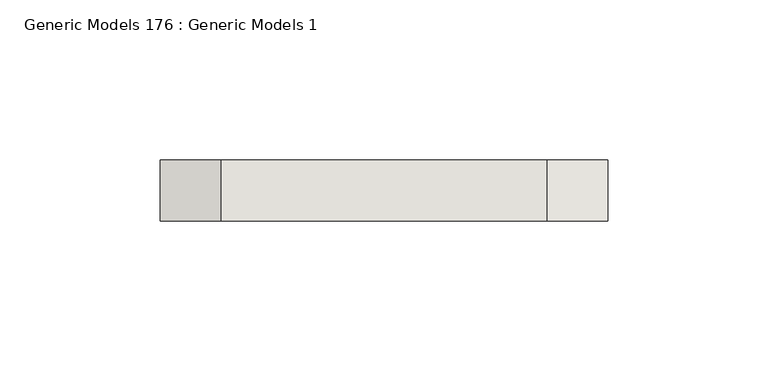
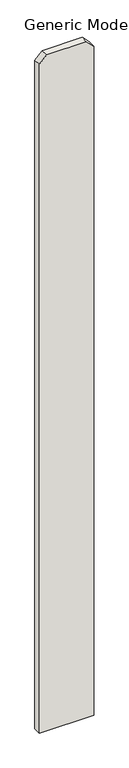
"""IFC4 building model written with IfcOpenShell, lengths in millimetres: wall geometry, Generic Models 176 : Generic Models 1."""

from ifc_helpers import new_model, si_unit, frame, origin, place, context, project, spatial, polyline, outline, extrude, source, transform, mapped, element, save


def generic_models_176_generic_models_1_2a1c1033(model_context):
    return source(origin(), model_context, "Body", "SweptSolid", [
        extrude(outline(polyline([(76.2, 325804.2125), (1885.95, 325804.2125), (1905.0, 325785.1625), (1905.0, 325683.5625), (1885.95, 325664.5125), (76.2, 325664.5125), (76.2, 325804.2125)])), frame((0.0, 547.6875, 0.0), z_axis=(0.0, 1.0, 0.0), x_axis=(0.0, 0.0, 1.0)), (0.0, 0.0, 1.0), 19.05),
    ])


if __name__ == "__main__":
    model = new_model("IFC4")
    model_context = context("Model", 3, world=origin())
    ifc_project = project(units=[si_unit("LENGTHUNIT", "METRE", prefix="MILLI")], contexts=[model_context])
    site = spatial("IfcSite", under=ifc_project)
    building = spatial("IfcBuilding", under=site)
    placement = place(None, origin())
    generic_models_176_generic_models_1_shape = generic_models_176_generic_models_1_2a1c1033(model_context)
    element("IfcWall", 1, ObjectType="Generic Models 176 : Generic Models 1", at=placement, inside=building, context=model_context, shape_type="MappedRepresentation", body=[
        mapped(generic_models_176_generic_models_1_shape, transform((0.0, 0.0, 0.0), x_axis=(1.0, 0.0, 0.0), y_axis=(0.0, 1.0, 0.0), z_axis=(0.0, 0.0, 1.0))),
    ])
    save(model, "model.ifc")

# Revit data of these elements
# Element 1 (IfcWall, "Generic Models 176 : Generic Models 1")
#   Materials on its faces: "VERTICAL 1X6 CEDAR PLANKS W/ CLEAR WOOD SEALER"
# Materials
#   "VERTICAL 1X6 CEDAR PLANKS W/ CLEAR WOOD SEALER": class "Wood", colour RGB 234 198 147, transparency 0, Description = "Pinus Echinata", Cost = 0
